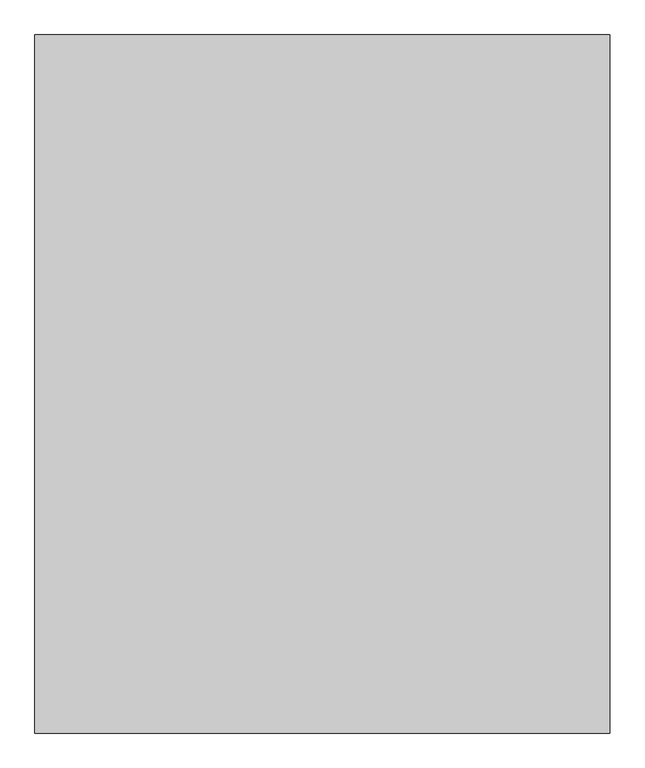
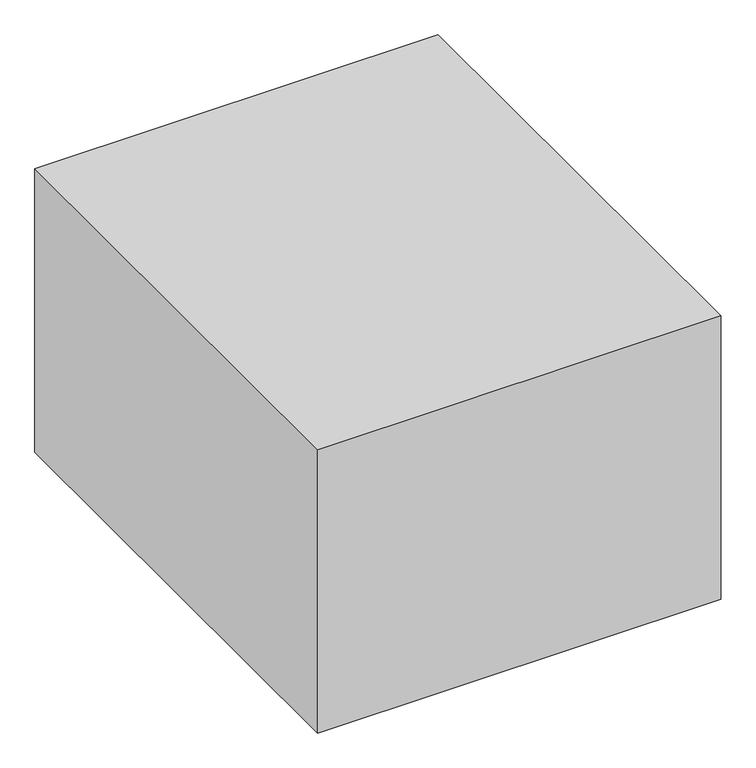
"""IFC4 building model written with IfcOpenShell, lengths in millimetres: proxy geometry, Space Planning Box_hec : Space Planning Box_hec."""

from ifc_helpers import new_model, si_unit, origin, origin_with_axes, place, context, project, spatial, polyline, outline, extrude, source, transform, mapped, element, save


def generic_models_235df1fa(model_context):
    return source(origin(), model_context, "Body", "SweptSolid", [
        extrude(outline(polyline([(3500.0, 4250.0), (3500.0, -4250.0), (-3500.0, -4250.0), (-3500.0, 4250.0), (3500.0, 4250.0)])), origin_with_axes(), (0.0, 0.0, 1.0), 5200.0),
    ])


if __name__ == "__main__":
    model = new_model("IFC4")
    model_context = context("Model", 3, world=origin())
    ifc_project = project(units=[si_unit("LENGTHUNIT", "METRE", prefix="MILLI")], contexts=[model_context])
    site = spatial("IfcSite", under=ifc_project)
    building = spatial("IfcBuilding", under=site)
    placement = place(None, origin())
    generic_models_shape = generic_models_235df1fa(model_context)
    element("IfcBuildingElementProxy", 1, Name="Space Planning Box_hec : Space Planning Box_hec", ObjectType="Space Planning Box_hec : Space Planning Box_hec", at=placement, inside=building, context=model_context, shape_type="MappedRepresentation", body=[
        mapped(generic_models_shape, transform((0.0, 0.0, 0.0), x_axis=(1.0, 0.0, 0.0), y_axis=(0.0, 1.0, 0.0), z_axis=(0.0, 0.0, 1.0))),
    ])
    save(model, "model.ifc")

# Revit data of these elements
# Type "Space Planning Box_hec : Space Planning Box_hec"
#   Type Comments = "..."
#   Room Name [instance default] = "?"
#   Interior Finish [instance default] = ""
#   Exterior Finish [instance default] = ""
#   Department [instance default] = ""
#   Assembly Code = "..."
#   ceiling height [instance default] = 0
#   Width [instance default] = 1524 mm
#   Program Area [instance default] = 0.00 m²
#   Length [instance default] = 1524 mm
#   Height [instance default] = 1524 mm
#   Area [instance default] = 2.32258 m²
#   Fill Color [instance default] = Cyan
#   Default Elevation = 0
# Element 1 (IfcBuildingElementProxy, "Space Planning Box_hec : Space Planning Box_hec")
#   Room Name = "Office-1"
#   Interior Finish = "IW1..N/A,,WB2..N/A,,FL6..N/A,,CL4..N/A"
#   Exterior Finish = "RF1..N/A,,EW1..N/A"
#   Department = "AR"
#   ceiling height = 2700
#   Width = 7000 mm
#   Program Area = 59.50 m²
#   Length = 8500 mm
#   Height = 5200 mm
#   Area = 59.50 m²
#   Materials on its faces: "Cyan"
# Materials
#   "Cyan": class "Generic", colour RGB 0 255 255, transparency 0.2, Cost = 0
